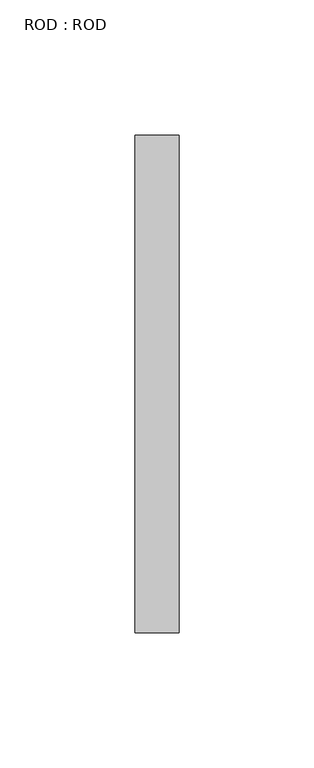
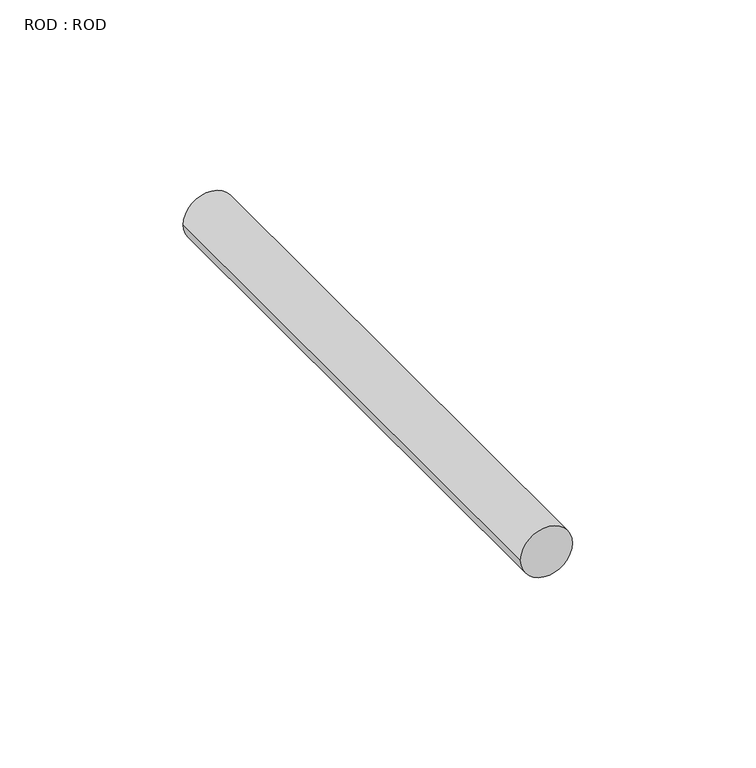
"""IFC4 building model written with IfcOpenShell, lengths in millimetres: proxy geometry, ROD : ROD."""

from ifc_helpers import new_model, si_unit, point, frame, origin, origin_2d, place, context, project, spatial, circle_curve, trimmed, segment, composite_curve, outline, extrude, source, transform, mapped, element, save


def rod_rod_9b827da6(model_context):
    return source(origin(), model_context, "Body", "SweptSolid", [
        extrude(outline(composite_curve([segment(trimmed(circle_curve(origin_2d(), 8.1359375), [point((0.0, 8.1359375))], [point((0.0, -8.1359375))], False, "CARTESIAN"), True, "CONTINUOUS"), segment(trimmed(circle_curve(origin_2d(), 8.1359375), [point((0.0, -8.1359375))], [point((0.0, 8.1359375))], False, "CARTESIAN"), True, "CONTINUOUS")], self_intersect=False)), frame((0.0, -152.4, 0.0), z_axis=(0.0, 1.0, 0.0), x_axis=(0.0, 0.0, 1.0)), (0.0, 0.0, 1.0), 184.15),
    ])


if __name__ == "__main__":
    model = new_model("IFC4")
    model_context = context("Model", 3, world=origin())
    ifc_project = project(units=[si_unit("LENGTHUNIT", "METRE", prefix="MILLI")], contexts=[model_context])
    site = spatial("IfcSite", under=ifc_project)
    building = spatial("IfcBuilding", under=site)
    placement = place(None, origin())
    rod_rod_shape = rod_rod_9b827da6(model_context)
    element("IfcBuildingElementProxy", 1, Name="ROD : ROD", ObjectType="ROD : ROD", at=placement, inside=building, context=model_context, shape_type="MappedRepresentation", body=[
        mapped(rod_rod_shape, transform((0.0, 0.0, 0.0), x_axis=(1.0, 0.0, 0.0), y_axis=(0.0, 1.0, 0.0), z_axis=(0.0, 0.0, 1.0))),
    ])
    save(model, "model.ifc")

# Revit data of these elements
# Type "ROD : ROD"
#   lenght = 0' - 7 1/4"
#   Radius = 0' - 0 41/128"
#   material [instance default] = 3/4" GALV. THRU BOLTS
# Materials
#   "3/4\" GALV. THRU BOLTS": class "Generic", colour RGB 105 69 171, transparency 0, Cost = 0
